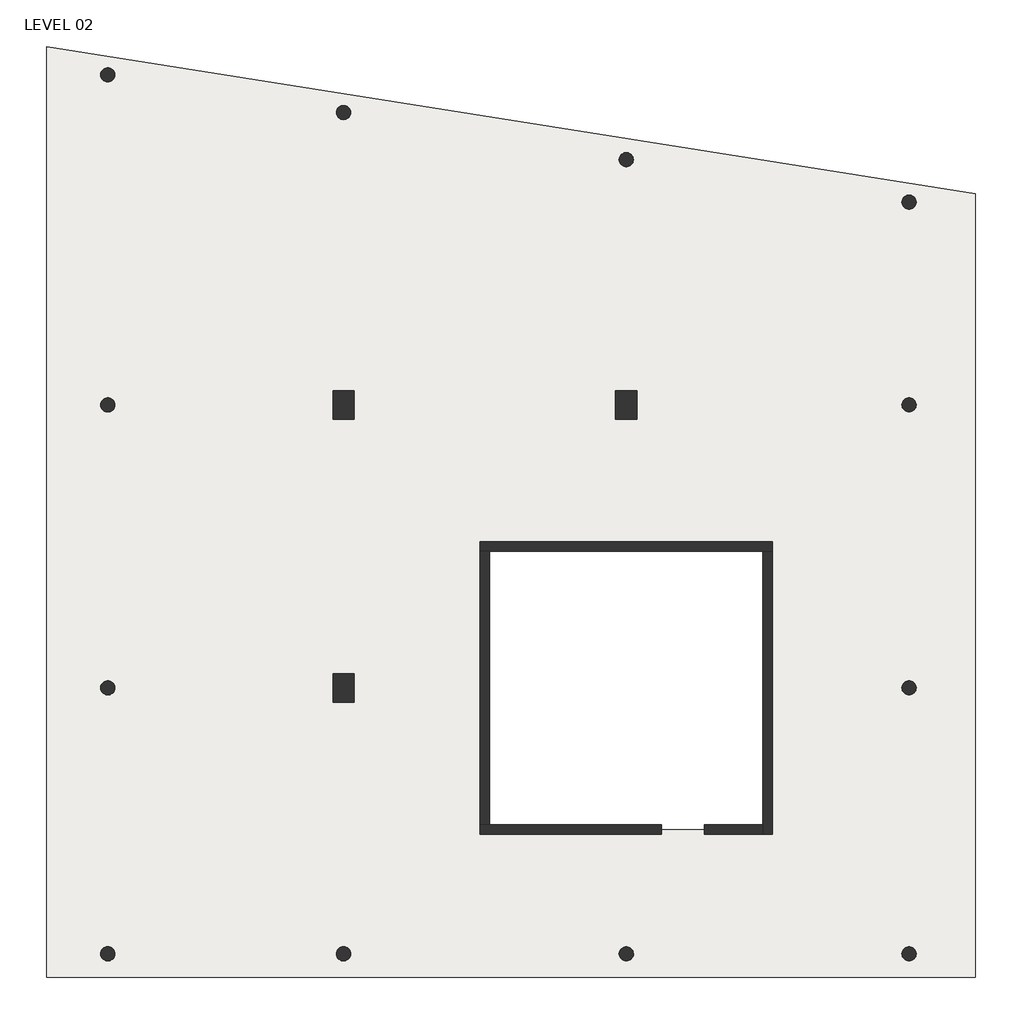
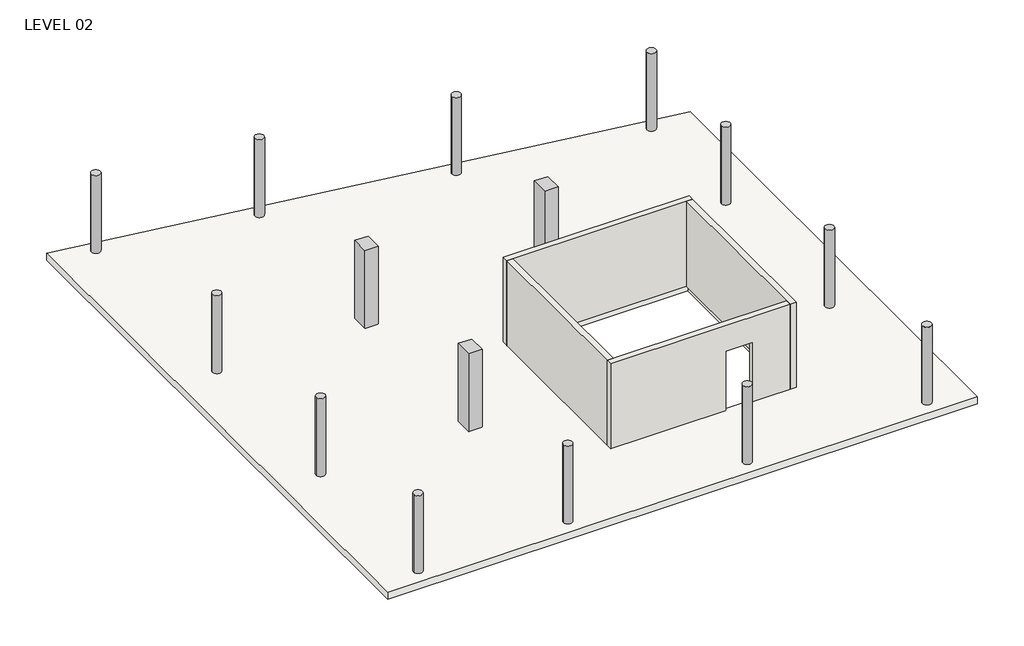
# One storey: 15 columns, 4 beams, 4 walls, 1 slab.
"""IFC4 building model written with IfcOpenShell, lengths in millimetres."""

import ifcopenshell
import ifcopenshell.guid

model = None  # the IFC model being written
_history = None  # IfcOwnerHistory: only IFC2X3 demands one
_inside = {}  # id of a spatial element -> (the spatial element, [elements in it])
_under = {}  # id of a project, library or spatial element -> (it, [spatial elements below it])
_declared = {}  # id of a project -> (the project, [libraries it declares])
_typed = {}  # id of a type object -> (the type object, [elements of that type])
_made_of = {}  # id of a material, layer set ... -> (it, [elements and type objects made of it])


def new_model(schema):
    """Start an empty IFC model of exactly this schema.

    Asked for "IFC4X3", IfcOpenShell would pick the latest addendum, in which some entities
    have other attributes; the version numbers below select the first issue.
    IFC2X3 requires an IfcOwnerHistory on every rooted entity: one is made here for all.
    """
    global model, _history
    if schema == "IFC4X3":
        model = ifcopenshell.file(schema_version=(4, 3, 0, 0))
    else:
        model = ifcopenshell.file(schema=schema)
    _inside.clear()
    _under.clear()
    _declared.clear()
    _typed.clear()
    _made_of.clear()
    _history = None
    if model.schema == "IFC2X3":
        org = make("IfcOrganization", Name="unknown")
        user = make(
            "IfcPersonAndOrganization",
            ThePerson=make("IfcPerson", FamilyName="unknown"),
            TheOrganization=org,
        )
        app = make(
            "IfcApplication",
            ApplicationDeveloper=org,
            Version="unknown",
            ApplicationFullName="unknown",
            ApplicationIdentifier="unknown",
        )
        _history = make(
            "IfcOwnerHistory",
            OwningUser=user,
            OwningApplication=app,
            ChangeAction="ADDED",
            CreationDate=0,
        )
    return model


def make(cls, **values):
    """One entity of the class cls with the attributes given. An attribute that is None is left unset."""
    return model.create_entity(
        cls, **{name: value for name, value in values.items() if value is not None}
    )


def rooted(cls, **values):
    """An entity with a GlobalId (a new one), such as an element, a storey or a relation."""
    return make(cls, GlobalId=ifcopenshell.guid.new(), OwnerHistory=_history, **values)


def si_unit(unit_type, name, prefix=None):
    """IfcSIUnit, for example si_unit("LENGTHUNIT", "METRE", prefix="MILLI")."""
    return make("IfcSIUnit", UnitType=unit_type, Prefix=prefix, Name=name)


def assignment(units):
    """IfcUnitAssignment: the units of a project."""
    return None if units is None else make("IfcUnitAssignment", Units=units)


def point(xyz):
    """IfcCartesianPoint."""
    return None if xyz is None else make("IfcCartesianPoint", Coordinates=xyz)


def direction(xyz):
    """IfcDirection."""
    return None if xyz is None else make("IfcDirection", DirectionRatios=xyz)


def frame(location, z_axis=None, x_axis=None):
    """IfcAxis2Placement3D, a coordinate frame: its origin and axes. An axis left out is left unset."""
    return make(
        "IfcAxis2Placement3D",
        Location=point(location),
        Axis=direction(z_axis),
        RefDirection=direction(x_axis),
    )


def frame_2d(location, x_axis=None):
    """IfcAxis2Placement2D, a coordinate frame in the plane: its origin and x axis."""
    return make(
        "IfcAxis2Placement2D", Location=point(location), RefDirection=direction(x_axis)
    )


def origin():
    """The frame at (0, 0, 0) with its axes left unset."""
    return frame((0.0, 0.0, 0.0))


def place(relative_to, where):
    """IfcLocalPlacement: puts the frame where relative to a parent placement (None: the world)."""
    return make(
        "IfcLocalPlacement", PlacementRelTo=relative_to, RelativePlacement=where
    )


def context(
    kind, dimensions, precision=None, world=None, true_north=None, identifier=None
):
    """IfcGeometricRepresentationContext, for example the 3D "Model" context."""
    return make(
        "IfcGeometricRepresentationContext",
        ContextIdentifier=identifier,
        ContextType=kind,
        CoordinateSpaceDimension=dimensions,
        Precision=precision,
        WorldCoordinateSystem=world,
        TrueNorth=true_north,
    )


def project(units=None, contexts=None):
    """IfcProject with its units and contexts."""
    return rooted(
        "IfcProject",
        Name="project",
        RepresentationContexts=contexts,
        UnitsInContext=assignment(units),
    )


def spatial(cls, under=None, at=None, **own):
    """A site, building, storey or space (cls), placed at a placement, below another one or the project."""
    s = rooted(cls, ObjectPlacement=at, **own)
    if under is not None:
        _under.setdefault(under.id(), (under, []))[1].append(s)
    return s


def polyline(points):
    """IfcPolyline through the points."""
    return make("IfcPolyline", Points=[point(p) for p in points])


def circle_curve(where, radius):
    """IfcCircle in the frame where."""
    return make("IfcCircle", Position=where, Radius=radius)


def trimmed(basis, trim1, trim2, sense, master):
    """IfcTrimmedCurve: the piece of a basis curve between two trims."""
    return make(
        "IfcTrimmedCurve",
        BasisCurve=basis,
        Trim1=trim1,
        Trim2=trim2,
        SenseAgreement=sense,
        MasterRepresentation=master,
    )


def segment(curve, same_sense, transition):
    """IfcCompositeCurveSegment."""
    return make(
        "IfcCompositeCurveSegment",
        Transition=transition,
        SameSense=same_sense,
        ParentCurve=curve,
    )


def composite_curve(segments, self_intersect=None):
    """IfcCompositeCurve: segments joined end to end."""
    return make("IfcCompositeCurve", Segments=segments, SelfIntersect=self_intersect)


def outline(outer, holes=None, kind="AREA"):
    """IfcArbitraryClosedProfileDef: a profile drawn as a closed curve; with holes, ...WithVoids."""
    if holes is None:
        return make("IfcArbitraryClosedProfileDef", ProfileType=kind, OuterCurve=outer)
    return make(
        "IfcArbitraryProfileDefWithVoids",
        ProfileType=kind,
        OuterCurve=outer,
        InnerCurves=holes,
    )


def extrude(swept, where, along, depth):
    """IfcExtrudedAreaSolid: the profile swept, set in the frame where, extruded along a direction by depth."""
    return make(
        "IfcExtrudedAreaSolid",
        SweptArea=swept,
        Position=where,
        ExtrudedDirection=direction(along),
        Depth=depth,
    )


def faces_of(points, faces, orient=None, outer=None):
    """IfcFace entities. A face is a list of loops; a loop is a list of indices into points, from 0.

    orient and outer hold one flag for each loop. By default every Orientation is true, the
    first loop of a face is its IfcFaceOuterBound and the others are IfcFaceBound.
    """
    made = []
    for i, loops in enumerate(faces):
        bounds = []
        for j, loop in enumerate(loops):
            is_outer = j == 0 if outer is None else outer[i][j]
            bounds.append(
                make(
                    "IfcFaceOuterBound" if is_outer else "IfcFaceBound",
                    Bound=make("IfcPolyLoop", Polygon=[points[k] for k in loop]),
                    Orientation=True if orient is None else orient[i][j],
                )
            )
        made.append(make("IfcFace", Bounds=bounds))
    return made


def faceted_brep(points, faces, orient=None, outer=None, voids=None):
    """IfcFacetedBrep: a solid bounded by flat faces; with voids (closed shells), ...WithVoids."""
    shared = [point(p) for p in points]
    hull = make("IfcClosedShell", CfsFaces=faces_of(shared, faces, orient, outer))
    if voids is None:
        return make("IfcFacetedBrep", Outer=hull)
    return make(
        "IfcFacetedBrepWithVoids",
        Outer=hull,
        Voids=[
            make(cls, CfsFaces=faces_of(shared, fs, o, b)) for cls, fs, o, b in voids
        ],
    )


def shape(context_of_items, identifier, shape_type, items):
    """IfcShapeRepresentation: the items that make up one representation, for example the "Body"."""
    return make(
        "IfcShapeRepresentation",
        ContextOfItems=context_of_items,
        RepresentationIdentifier=identifier,
        RepresentationType=shape_type,
        Items=items,
    )


def made_of(thing, what):
    """Note that an element or type object is made of a material, layer set ...; save() writes the relation."""
    if what is not None:
        _made_of.setdefault(what.id(), (what, []))[1].append(thing)
    return thing


def element(
    cls,
    number,
    at=None,
    inside=None,
    cuts=None,
    type_object=None,
    material=None,
    context=None,
    identifier="Body",
    shape_type=None,
    held_by="IfcProductDefinitionShape",
    body=None,
    shapes=None,
    **own,
):
    """One element of the class cls, such as IfcWall. Its Tag is "e" and its number.

    at: its placement. inside: the storey or other place that contains it. cuts: it is an
    opening in that element (IfcRelVoidsElement). A single representation is given by context,
    identifier, shape_type and body (its items); several are given by shapes. held_by: the class
    of the entity that holds the representations. save() writes the other relations.
    """
    e = rooted(cls, Tag="e%d" % number, ObjectPlacement=at, **own)
    if body is not None:
        shapes = [shape(context, identifier, shape_type, body)]
    if shapes is not None:
        e.Representation = make(held_by, Representations=shapes)
    if inside is not None:
        _inside.setdefault(inside.id(), (inside, []))[1].append(e)
    if cuts is not None:
        rooted(
            "IfcRelVoidsElement", RelatingBuildingElement=cuts, RelatedOpeningElement=e
        )
    if type_object is not None:
        _typed.setdefault(type_object.id(), (type_object, []))[1].append(e)
    return made_of(e, material)


def aggregate(whole, parts):
    """IfcRelAggregates: a whole, such as a stair, and the parts it consists of."""
    return rooted("IfcRelAggregates", RelatingObject=whole, RelatedObjects=parts)


def save(model, path):
    """Write the relations noted so far, then the file.

    IfcRelAggregates (storeys below a building ...), IfcRelContainedInSpatialStructure (elements
    in a storey), IfcRelDefinesByType, IfcRelAssociatesMaterial and IfcRelDeclares: one each for
    every whole, place, type object, material and project.
    """
    for whole, parts in _under.values():
        aggregate(whole, parts)
    for where, things in _inside.values():
        rooted(
            "IfcRelContainedInSpatialStructure",
            RelatedElements=things,
            RelatingStructure=where,
        )
    for kind, things in _typed.values():
        rooted("IfcRelDefinesByType", RelatedObjects=things, RelatingType=kind)
    for what, things in _made_of.values():
        rooted("IfcRelAssociatesMaterial", RelatedObjects=things, RelatingMaterial=what)
    for by, libraries in _declared.values():
        rooted("IfcRelDeclares", RelatingContext=by, RelatedDefinitions=libraries)
    model.write(path)


model = new_model("IFC4")

# Units and contexts
model_context = context("Model", 3, world=origin())
ifc_project = project(units=[si_unit("LENGTHUNIT", "METRE", prefix="MILLI")], contexts=[model_context])

# Site, building, storey
site = spatial("IfcSite", under=ifc_project)
building = spatial("IfcBuilding", under=site)
storey = spatial("IfcBuildingStorey", under=building, Name="LEVEL 02", Elevation=6000.0)

# Beams
placement = place(None, origin())
element("IfcBeam", 1, ObjectType="BHm_StructuralFraming_Concrete-RectangularBeam : 300x500 DP RC BEAM", at=placement, inside=storey, context=model_context, shape_type="SweptSolid", body=[
    extrude(outline(composite_curve([segment(polyline([(-15925.1680269, 21640.7845261), (-15925.1680269, 14640.7845261)]), True, "CONTINUOUS"), segment(trimmed(circle_curve(frame_2d((-16075.1680269, 14640.7845261)), 150.0), [point((-15925.1680269, 14640.7845261))], [point((-16225.1680269, 14640.7845261))], True, "CARTESIAN"), True, "CONTINUOUS"), segment(polyline([(-16225.1680269, 14640.7845261), (-16225.1680269, 21640.7845261)]), True, "CONTINUOUS"), segment(trimmed(circle_curve(frame_2d((-16075.1680269, 21640.7845261)), 150.0), [point((-16225.1680269, 21640.7845261))], [point((-15925.1680269, 21640.7845261))], True, "CARTESIAN"), True, "CONTINUOUS")], self_intersect=False)), frame((0.0, 0.0, 5500.0), z_axis=(0.0, 0.0, 1.0), x_axis=(1.0, 0.0, 0.0)), (0.0, 0.0, 1.0), 250.0),
])
element("IfcBeam", 2, ObjectType="BHm_StructuralFraming_Concrete-RectangularBeam : 300x500 DP RC BEAM", at=placement, inside=storey, context=model_context, shape_type="SweptSolid", body=[
    extrude(outline(composite_curve([segment(polyline([(-10925.1680269, 20840.7845261), (-10925.1680269, 14940.7845261), (-11225.1680269, 14940.7845261), (-11225.1680269, 20840.7845261)]), True, "CONTINUOUS"), segment(trimmed(circle_curve(frame_2d((-11075.1680269, 20840.7845261)), 150.0), [point((-11225.1680269, 20840.7845261))], [point((-10925.1680269, 20840.7845261))], True, "CARTESIAN"), True, "CONTINUOUS")], self_intersect=False)), frame((0.0, 0.0, 5500.0), z_axis=(0.0, 0.0, 1.0), x_axis=(1.0, 0.0, 0.0)), (0.0, 0.0, 1.0), 250.0),
])
element("IfcBeam", 3, ObjectType="BHm_StructuralFraming_Concrete-RectangularBeam : 300x500 DP RC BEAM", at=placement, inside=storey, context=model_context, shape_type="SweptSolid", body=[
    extrude(outline(composite_curve([segment(polyline([(-4925.1680269, 19840.7845261), (-4925.1680269, 14940.7845261), (-5225.1680269, 14940.7845261), (-5225.1680269, 19840.7845261)]), True, "CONTINUOUS"), segment(trimmed(circle_curve(frame_2d((-5075.1680269, 19840.7845261)), 150.0), [point((-5225.1680269, 19840.7845261))], [point((-4925.1680269, 19840.7845261))], True, "CARTESIAN"), True, "CONTINUOUS")], self_intersect=False)), frame((0.0, 0.0, 5500.0), z_axis=(0.0, 0.0, 1.0), x_axis=(1.0, 0.0, 0.0)), (0.0, 0.0, 1.0), 250.0),
])
element("IfcBeam", 4, ObjectType="BHm_StructuralFraming_Concrete-RectangularBeam : 300x500 DP RC BEAM", at=placement, inside=storey, context=model_context, shape_type="SweptSolid", body=[
    extrude(outline(composite_curve([segment(polyline([(1074.8319731, 18940.7845261), (1074.8319731, 14640.7845261)]), True, "CONTINUOUS"), segment(trimmed(circle_curve(frame_2d((924.8319731, 14640.7845261)), 150.0), [point((1074.8319731, 14640.7845261))], [point((774.8319731, 14640.7845261))], True, "CARTESIAN"), True, "CONTINUOUS"), segment(polyline([(774.8319731, 14640.7845261), (774.8319731, 18940.7845261)]), True, "CONTINUOUS"), segment(trimmed(circle_curve(frame_2d((924.8319731, 18940.7845261)), 150.0), [point((774.8319731, 18940.7845261))], [point((1074.8319731, 18940.7845261))], True, "CARTESIAN"), True, "CONTINUOUS")], self_intersect=False)), frame((0.0, 0.0, 5500.0), z_axis=(0.0, 0.0, 1.0), x_axis=(1.0, 0.0, 0.0)), (0.0, 0.0, 1.0), 250.0),
])

# Columns
element("IfcColumn", 5, ObjectType="BHm_StructuralColumns_ConcreteRound : 300 Ø RC COL", at=placement, inside=storey, context=model_context, shape_type="SweptSolid", body=[
    extrude(outline(composite_curve([segment(trimmed(circle_curve(frame_2d((-5075.1680269, 3000.0)), 150.0), [point((-5225.1680269, 3000.0))], [point((-4925.1680269, 3000.0))], False, "CARTESIAN"), True, "CONTINUOUS"), segment(trimmed(circle_curve(frame_2d((-5075.1680269, 3000.0)), 150.0), [point((-4925.1680269, 3000.0))], [point((-5225.1680269, 3000.0))], False, "CARTESIAN"), True, "CONTINUOUS")], self_intersect=False)), frame((0.0, 0.0, 6000.0), z_axis=(0.0, 0.0, 1.0), x_axis=(1.0, 0.0, 0.0)), (0.0, 0.0, 1.0), 2750.0),
])
element("IfcColumn", 6, ObjectType="BHm_StructuralColumns_ConcreteRound : 300 Ø RC COL", at=placement, inside=storey, context=model_context, shape_type="SweptSolid", body=[
    extrude(outline(composite_curve([segment(trimmed(circle_curve(frame_2d((924.8319731, 14640.7845261)), 150.0), [point((774.8319731, 14640.7845261))], [point((1074.8319731, 14640.7845261))], False, "CARTESIAN"), True, "CONTINUOUS"), segment(trimmed(circle_curve(frame_2d((924.8319731, 14640.7845261)), 150.0), [point((1074.8319731, 14640.7845261))], [point((774.8319731, 14640.7845261))], False, "CARTESIAN"), True, "CONTINUOUS")], self_intersect=False)), frame((0.0, 0.0, 6000.0), z_axis=(0.0, 0.0, 1.0), x_axis=(1.0, 0.0, 0.0)), (0.0, 0.0, 1.0), 2750.0),
])
element("IfcColumn", 7, ObjectType="BHm_StructuralColumns_ConcreteRound : 300 Ø RC COL", at=placement, inside=storey, context=model_context, shape_type="SweptSolid", body=[
    extrude(outline(composite_curve([segment(trimmed(circle_curve(frame_2d((924.8319731, 8640.7845261)), 150.0), [point((774.8319731, 8640.7845261))], [point((1074.8319731, 8640.7845261))], False, "CARTESIAN"), True, "CONTINUOUS"), segment(trimmed(circle_curve(frame_2d((924.8319731, 8640.7845261)), 150.0), [point((1074.8319731, 8640.7845261))], [point((774.8319731, 8640.7845261))], False, "CARTESIAN"), True, "CONTINUOUS")], self_intersect=False)), frame((0.0, 0.0, 6000.0), z_axis=(0.0, 0.0, 1.0), x_axis=(1.0, 0.0, 0.0)), (0.0, 0.0, 1.0), 2750.0),
])
element("IfcColumn", 8, ObjectType="BHm_StructuralColumns_ConcreteRound : 300 Ø RC COL", at=placement, inside=storey, context=model_context, shape_type="SweptSolid", body=[
    extrude(outline(composite_curve([segment(trimmed(circle_curve(frame_2d((924.8319731, 3000.0)), 150.0), [point((774.8319731, 3000.0))], [point((1074.8319731, 3000.0))], False, "CARTESIAN"), True, "CONTINUOUS"), segment(trimmed(circle_curve(frame_2d((924.8319731, 3000.0)), 150.0), [point((1074.8319731, 3000.0))], [point((774.8319731, 3000.0))], False, "CARTESIAN"), True, "CONTINUOUS")], self_intersect=False)), frame((0.0, 0.0, 6000.0), z_axis=(0.0, 0.0, 1.0), x_axis=(1.0, 0.0, 0.0)), (0.0, 0.0, 1.0), 2750.0),
])
element("IfcColumn", 9, ObjectType="BHm_StructuralColumns_ConcreteRound : 300 Ø RC COL", at=placement, inside=storey, context=model_context, shape_type="SweptSolid", body=[
    extrude(outline(composite_curve([segment(trimmed(circle_curve(frame_2d((-11075.1680269, 3000.0)), 150.0), [point((-11225.1680269, 3000.0))], [point((-10925.1680269, 3000.0))], False, "CARTESIAN"), True, "CONTINUOUS"), segment(trimmed(circle_curve(frame_2d((-11075.1680269, 3000.0)), 150.0), [point((-10925.1680269, 3000.0))], [point((-11225.1680269, 3000.0))], False, "CARTESIAN"), True, "CONTINUOUS")], self_intersect=False)), frame((0.0, 0.0, 6000.0), z_axis=(0.0, 0.0, 1.0), x_axis=(1.0, 0.0, 0.0)), (0.0, 0.0, 1.0), 2750.0),
])
element("IfcColumn", 10, ObjectType="BHm_StructuralColumns_ConcreteRound : 300 Ø RC COL", at=placement, inside=storey, context=model_context, shape_type="SweptSolid", body=[
    extrude(outline(composite_curve([segment(trimmed(circle_curve(frame_2d((-16075.1680269, 14640.7845261)), 150.0), [point((-16225.1680269, 14640.7845261))], [point((-15925.1680269, 14640.7845261))], False, "CARTESIAN"), True, "CONTINUOUS"), segment(trimmed(circle_curve(frame_2d((-16075.1680269, 14640.7845261)), 150.0), [point((-15925.1680269, 14640.7845261))], [point((-16225.1680269, 14640.7845261))], False, "CARTESIAN"), True, "CONTINUOUS")], self_intersect=False)), frame((0.0, 0.0, 6000.0), z_axis=(0.0, 0.0, 1.0), x_axis=(1.0, 0.0, 0.0)), (0.0, 0.0, 1.0), 2750.0),
])
element("IfcColumn", 11, ObjectType="BHm_StructuralColumns_ConcreteRound : 300 Ø RC COL", at=placement, inside=storey, context=model_context, shape_type="SweptSolid", body=[
    extrude(outline(composite_curve([segment(trimmed(circle_curve(frame_2d((-16075.1680269, 8640.7845261)), 150.0), [point((-16225.1680269, 8640.7845261))], [point((-15925.1680269, 8640.7845261))], False, "CARTESIAN"), True, "CONTINUOUS"), segment(trimmed(circle_curve(frame_2d((-16075.1680269, 8640.7845261)), 150.0), [point((-15925.1680269, 8640.7845261))], [point((-16225.1680269, 8640.7845261))], False, "CARTESIAN"), True, "CONTINUOUS")], self_intersect=False)), frame((0.0, 0.0, 6000.0), z_axis=(0.0, 0.0, 1.0), x_axis=(1.0, 0.0, 0.0)), (0.0, 0.0, 1.0), 2750.0),
])
element("IfcColumn", 12, ObjectType="BHm_StructuralColumns_ConcreteRound : 300 Ø RC COL", at=placement, inside=storey, context=model_context, shape_type="SweptSolid", body=[
    extrude(outline(composite_curve([segment(trimmed(circle_curve(frame_2d((-16075.1680269, 3000.0)), 150.0), [point((-16225.1680269, 3000.0))], [point((-15925.1680269, 3000.0))], False, "CARTESIAN"), True, "CONTINUOUS"), segment(trimmed(circle_curve(frame_2d((-16075.1680269, 3000.0)), 150.0), [point((-15925.1680269, 3000.0))], [point((-16225.1680269, 3000.0))], False, "CARTESIAN"), True, "CONTINUOUS")], self_intersect=False)), frame((0.0, 0.0, 6000.0), z_axis=(0.0, 0.0, 1.0), x_axis=(1.0, 0.0, 0.0)), (0.0, 0.0, 1.0), 2750.0),
])
element("IfcColumn", 13, ObjectType="BHm_StructuralColumns_ConcreteRound : 300 Ø RC COL", at=placement, inside=storey, context=model_context, shape_type="SweptSolid", body=[
    extrude(outline(composite_curve([segment(trimmed(circle_curve(frame_2d((-11075.1680269, 20840.7845261)), 150.0), [point((-11225.1680269, 20840.7845261))], [point((-10925.1680269, 20840.7845261))], False, "CARTESIAN"), True, "CONTINUOUS"), segment(trimmed(circle_curve(frame_2d((-11075.1680269, 20840.7845261)), 150.0), [point((-10925.1680269, 20840.7845261))], [point((-11225.1680269, 20840.7845261))], False, "CARTESIAN"), True, "CONTINUOUS")], self_intersect=False)), frame((0.0, 0.0, 6000.0), z_axis=(0.0, 0.0, 1.0), x_axis=(1.0, 0.0, 0.0)), (0.0, 0.0, 1.0), 2750.0),
])
element("IfcColumn", 14, ObjectType="BHm_StructuralColumns_ConcreteRound : 300 Ø RC COL", at=placement, inside=storey, context=model_context, shape_type="SweptSolid", body=[
    extrude(outline(composite_curve([segment(trimmed(circle_curve(frame_2d((-5075.1680269, 19840.7845261)), 150.0), [point((-5225.1680269, 19840.7845261))], [point((-4925.1680269, 19840.7845261))], False, "CARTESIAN"), True, "CONTINUOUS"), segment(trimmed(circle_curve(frame_2d((-5075.1680269, 19840.7845261)), 150.0), [point((-4925.1680269, 19840.7845261))], [point((-5225.1680269, 19840.7845261))], False, "CARTESIAN"), True, "CONTINUOUS")], self_intersect=False)), frame((0.0, 0.0, 6000.0), z_axis=(0.0, 0.0, 1.0), x_axis=(1.0, 0.0, 0.0)), (0.0, 0.0, 1.0), 2750.0),
])
element("IfcColumn", 15, ObjectType="BHm_StructuralColumns_ConcreteRound : 300 Ø RC COL", at=placement, inside=storey, context=model_context, shape_type="SweptSolid", body=[
    extrude(outline(composite_curve([segment(trimmed(circle_curve(frame_2d((924.8319731, 18940.7845261)), 150.0), [point((774.8319731, 18940.7845261))], [point((1074.8319731, 18940.7845261))], False, "CARTESIAN"), True, "CONTINUOUS"), segment(trimmed(circle_curve(frame_2d((924.8319731, 18940.7845261)), 150.0), [point((1074.8319731, 18940.7845261))], [point((774.8319731, 18940.7845261))], False, "CARTESIAN"), True, "CONTINUOUS")], self_intersect=False)), frame((0.0, 0.0, 6000.0), z_axis=(0.0, 0.0, 1.0), x_axis=(1.0, 0.0, 0.0)), (0.0, 0.0, 1.0), 2750.0),
])
element("IfcColumn", 16, ObjectType="BHm_StructuralColumns_ConcreteRound : 300 Ø RC COL", at=placement, inside=storey, context=model_context, shape_type="SweptSolid", body=[
    extrude(outline(composite_curve([segment(trimmed(circle_curve(frame_2d((-16075.1680269, 21640.7845261)), 150.0), [point((-16225.1680269, 21640.7845261))], [point((-15925.1680269, 21640.7845261))], False, "CARTESIAN"), True, "CONTINUOUS"), segment(trimmed(circle_curve(frame_2d((-16075.1680269, 21640.7845261)), 150.0), [point((-15925.1680269, 21640.7845261))], [point((-16225.1680269, 21640.7845261))], False, "CARTESIAN"), True, "CONTINUOUS")], self_intersect=False)), frame((0.0, 0.0, 6000.0), z_axis=(0.0, 0.0, 1.0), x_axis=(1.0, 0.0, 0.0)), (0.0, 0.0, 1.0), 2750.0),
])
element("IfcColumn", 17, ObjectType="BHm_StructuralColumns_ConcreteRectangular : 450x600 RC COL", at=placement, inside=storey, context=model_context, shape_type="SweptSolid", body=[
    extrude(outline(polyline([(-10850.1680269, 14940.7845261), (-10850.1680269, 14340.7845261), (-11300.1680269, 14340.7845261), (-11300.1680269, 14940.7845261), (-10850.1680269, 14940.7845261)])), frame((0.0, 0.0, 6000.0), z_axis=(0.0, 0.0, 1.0), x_axis=(1.0, 0.0, 0.0)), (0.0, 0.0, 1.0), 2750.0),
])
element("IfcColumn", 18, ObjectType="BHm_StructuralColumns_ConcreteRectangular : 450x600 RC COL", at=placement, inside=storey, context=model_context, shape_type="SweptSolid", body=[
    extrude(outline(polyline([(-10850.1680269, 8940.7845261), (-10850.1680269, 8340.7845261), (-11300.1680269, 8340.7845261), (-11300.1680269, 8940.7845261), (-10850.1680269, 8940.7845261)])), frame((0.0, 0.0, 6000.0), z_axis=(0.0, 0.0, 1.0), x_axis=(1.0, 0.0, 0.0)), (0.0, 0.0, 1.0), 2750.0),
])
element("IfcColumn", 19, ObjectType="BHm_StructuralColumns_ConcreteRectangular : 450x600 RC COL", at=placement, inside=storey, context=model_context, shape_type="SweptSolid", body=[
    extrude(outline(polyline([(-4850.1680269, 14940.7845261), (-4850.1680269, 14340.7845261), (-5300.1680269, 14340.7845261), (-5300.1680269, 14940.7845261), (-4850.1680269, 14940.7845261)])), frame((0.0, 0.0, 6000.0), z_axis=(0.0, 0.0, 1.0), x_axis=(1.0, 0.0, 0.0)), (0.0, 0.0, 1.0), 2750.0),
])

# Slab
element("IfcSlab", 20, ObjectType="250 THK RC SLAB", at=placement, inside=storey, context=model_context, shape_type="SweptSolid", body=[
    extrude(outline(polyline([(2324.8319731, 19120.6110517), (2324.8319731, 2500.0), (-17375.1680269, 2500.0), (-17375.1680269, 22240.7845261), (2324.8319731, 19120.6110517)]), holes=[polyline([(-2075.1680269, 11640.7845261), (-8075.1680269, 11640.7845261), (-8075.1680269, 5640.7845261), (-2075.1680269, 5640.7845261), (-2075.1680269, 11640.7845261)])]), frame((0.0, 0.0, 5750.0), z_axis=(0.0, 0.0, 1.0), x_axis=(1.0, 0.0, 0.0)), (0.0, 0.0, 1.0), 250.0),
])

# Walls
element("IfcWall", 21, ObjectType="200 THK R.C. WALL", at=placement, inside=storey, context=model_context, shape_type="Brep", body=[
    faceted_brep([(-8175.1680269, 11540.7845261, 6000.0), (-7975.1680269, 11540.7845261, 6000.0), (-2175.1680269, 11540.7845261, 6000.0), (-1975.1680269, 11540.7845261, 6000.0), (-1975.1680269, 11540.7845261, 9000.0), (-2175.1680269, 11540.7845261, 9000.0), (-7975.1680269, 11540.7845261, 9000.0), (-8175.1680269, 11540.7845261, 9000.0), (-8175.1680269, 11740.7845261, 6000.0), (-8175.1680269, 11740.7845261, 9000.0), (-1975.1680269, 11740.7845261, 9000.0), (-1975.1680269, 11740.7845261, 6000.0)], [[[0, 1, 2, 3, 4, 5, 6, 7]], [[8, 9, 10, 11]], [[3, 2, 1, 0, 8, 11]], [[7, 6, 5, 4, 10, 9]], [[4, 3, 11, 10]], [[0, 7, 9, 8]]]),
])
element("IfcWall", 22, ObjectType="200 THK R.C. WALL", at=placement, inside=storey, context=model_context, shape_type="Brep", body=[
    faceted_brep([(-2175.1680269, 11540.7845261, 6000.0), (-2175.1680269, 5740.7845261, 6000.0), (-2175.1680269, 5540.7845261, 6000.0), (-2175.1680269, 5540.7845261, 9000.0), (-2175.1680269, 5740.7845261, 9000.0), (-2175.1680269, 11540.7845261, 9000.0), (-1975.1680269, 11540.7845261, 6000.0), (-1975.1680269, 11540.7845261, 9000.0), (-1975.1680269, 5540.7845261, 9000.0), (-1975.1680269, 5540.7845261, 6000.0)], [[[0, 1, 2, 3, 4, 5]], [[6, 7, 8, 9]], [[2, 1, 0, 6, 9]], [[5, 4, 3, 8, 7]], [[0, 5, 7, 6]], [[3, 2, 9, 8]]]),
])
element("IfcWall", 23, ObjectType="200 THK R.C. WALL", at=placement, inside=storey, context=model_context, shape_type="Brep", body=[
    faceted_brep([(-2175.1680269, 5740.7845261, 6000.0), (-3417.6680269, 5740.7845261, 6000.0), (-3417.6680269, 5740.7845261, 8100.0), (-4332.6680269, 5740.7845261, 8100.0), (-4332.6680269, 5740.7845261, 6000.0), (-7975.1680269, 5740.7845261, 6000.0), (-8175.1680269, 5740.7845261, 6000.0), (-8175.1680269, 5740.7845261, 9000.0), (-7975.1680269, 5740.7845261, 9000.0), (-2175.1680269, 5740.7845261, 9000.0), (-3417.6680269, 5540.7845261, 8100.0), (-3417.6680269, 5540.7845261, 6000.0), (-2175.1680269, 5540.7845261, 6000.0), (-2175.1680269, 5540.7845261, 9000.0), (-8175.1680269, 5540.7845261, 9000.0), (-8175.1680269, 5540.7845261, 6000.0), (-4332.6680269, 5540.7845261, 6000.0), (-4332.6680269, 5540.7845261, 8100.0)], [[[0, 1, 2, 3, 4, 5, 6, 7, 8, 9]], [[10, 11, 12, 13, 14, 15, 16, 17]], [[16, 15, 6, 5, 4]], [[12, 11, 1, 0]], [[9, 8, 7, 14, 13]], [[0, 9, 13, 12]], [[7, 6, 15, 14]], [[4, 3, 17, 16]], [[2, 1, 11, 10]], [[3, 2, 10, 17]]]),
])
element("IfcWall", 24, ObjectType="200 THK R.C. WALL", at=placement, inside=storey, context=model_context, shape_type="SweptSolid", body=[
    extrude(outline(polyline([(-7975.1680269, 11540.7845261), (-7975.1680269, 5740.7845261), (-8175.1680269, 5740.7845261), (-8175.1680269, 11540.7845261), (-7975.1680269, 11540.7845261)])), frame((0.0, 0.0, 6000.0), z_axis=(0.0, 0.0, 1.0), x_axis=(1.0, 0.0, 0.0)), (0.0, 0.0, 1.0), 3000.0),
])

save(model, "model.ifc")

# Revit data of these elements
# Type "BHm_StructuralFraming_Concrete-RectangularBeam : 300x500 DP RC BEAM"
#   Keynote = "E"
#   BHE_Width = 300.000 mm
#   BHE_Length [instance default] = 1524.000 mm
#   BHE_Height = 500.000 mm
#   Length [instance default] = 1524.000 mm
#   b = 300.000 mm
#   h = 500.000 mm
#   Structural Material [instance default] = none
#   Assembly Code = ""
# Type "BHm_StructuralColumns_ConcreteRound : 300 Ø RC COL"
#   Keynote = "E"
#   b = 300.000 mm
#   BHE_Length [instance default] = 2500.000 mm
#   BHE_Diameter = 300.000 mm
#   Structural Material [instance default] = none
# Type "BHm_StructuralColumns_ConcreteRectangular : 450x600 RC COL"
#   Keynote = "E"
#   b = 450.000 mm
#   h = 600.000 mm
#   BHE_Width = 450.000 mm
#   BHE_Length [instance default] = 2500.000 mm
#   BHE_Height = 600.000 mm
#   Structural Material [instance default] = none
# Type "250 THK RC SLAB"
#   Function = 0
#   Layers, outside or top first: 250.000 mm "BHE_Concrete - Cast In-Place" (function 1)
# Type "200 THK R.C. WALL"
#   Layers, outside or top first: 200.000 mm "BHE_Concrete - Cast In-Place" (function 1)
# Element 1 (IfcBeam, "BHm_StructuralFraming_Concrete-RectangularBeam : 300x500 DP RC BEAM")
#   Comments = ""
#   BHE_Length = 7000.000 mm
#   Structural Material = none
#   Phase Created = New Construction
#   Materials on its faces: "BHE_Concrete - Cast In-Place"
# Element 2 (IfcBeam, "BHm_StructuralFraming_Concrete-RectangularBeam : 300x500 DP RC BEAM")
#   Comments = ""
#   BHE_Length = 6200.000 mm
#   Structural Material = none
#   Phase Created = New Construction
#   Materials on its faces: "BHE_Concrete - Cast In-Place"
# Element 3 (IfcBeam, "BHm_StructuralFraming_Concrete-RectangularBeam : 300x500 DP RC BEAM")
#   Comments = ""
#   BHE_Length = 5200.000 mm
#   Structural Material = none
#   Phase Created = New Construction
#   Materials on its faces: "BHE_Concrete - Cast In-Place"
# Element 4 (IfcBeam, "BHm_StructuralFraming_Concrete-RectangularBeam : 300x500 DP RC BEAM")
#   Comments = ""
#   BHE_Length = 4300.000 mm
#   Structural Material = none
#   Phase Created = New Construction
#   Materials on its faces: "BHE_Concrete - Cast In-Place"
# Elements 5, 6, 7, 8, 9, 10, 11, 12, 13, 14, 15, 16 (IfcColumn, "BHm_StructuralColumns_ConcreteRound : 300 Ø RC COL")
#   Comments = ""
#   Structural Material = none
#   Phase Created = New Construction
#   Materials on its faces: "BHE_Concrete - Cast In-Place"
# Elements 17, 18, 19 (IfcColumn, "BHm_StructuralColumns_ConcreteRectangular : 450x600 RC COL")
#   Comments = ""
#   Structural Material = none
#   Phase Created = New Construction
#   Materials on its faces: "BHE_Concrete - Cast In-Place"
# Element 20 (IfcSlab, "250 THK RC SLAB")
#   Comments = ""
#   built-in parameter 1001955 = -0.15708 (stored number, unit not read)
#   Height Offset From Level = 0.000 mm
#   built-in parameter 1001954 = 1
#   Phase Created = New Construction
#   Materials on its faces: "BHE_Concrete - Cast In-Place"
# Elements 21, 22, 23, 24 (IfcWall, "200 THK R.C. WALL")
#   Comments = ""
#   Top Offset = 0.000 mm
#   Base Offset = 0.000 mm
#   wall height = 3000.000 mm
#   Phase Created = New Construction
#   Base Constraint = LEVEL 02
#   Top Constraint = LEVEL 03
#   Materials on its faces: "BHE_Concrete - Cast In-Place"
# Materials
#   "BHE_Concrete - Cast In-Place": class "Concrete", colour RGB 192 192 192, transparency 0, Cost = 0
